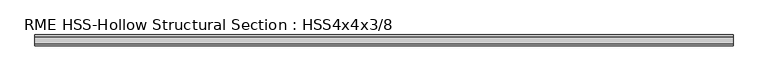
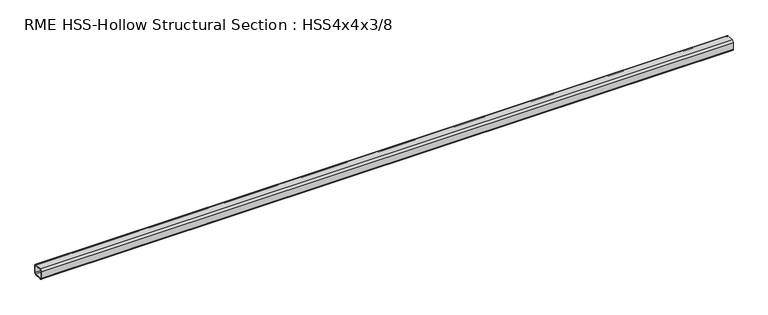
"""IFC4 building model written with IfcOpenShell, lengths in millimetres: member geometry, RME HSS-Hollow Structural Section : HSS4x4x3/8."""

from ifc_helpers import new_model, si_unit, point, frame, frame_2d, origin, place, context, project, spatial, polyline, circle_curve, trimmed, segment, composite_curve, outline, extrude, source, transform, mapped, element, save


def rme_hss_hollow_structural_section_hss4x4x3_8_4a4d7d68(model_context):
    return source(origin(), model_context, "Body", "SweptSolid", [
        extrude(outline(composite_curve([segment(polyline([(50.8, 33.0708), (50.8, -33.0708)]), True, "CONTINUOUS"), segment(trimmed(circle_curve(frame_2d((33.0708, -33.0708)), 17.7292), [point((50.8, -33.0708))], [point((33.0708, -50.8))], False, "CARTESIAN"), True, "CONTINUOUS"), segment(polyline([(33.0708, -50.8), (-33.0708, -50.8)]), True, "CONTINUOUS"), segment(trimmed(circle_curve(frame_2d((-33.0708, -33.0708)), 17.7292), [point((-33.0708, -50.8))], [point((-50.8, -33.0708))], False, "CARTESIAN"), True, "CONTINUOUS"), segment(polyline([(-50.8, -33.0708), (-50.8, 33.0708)]), True, "CONTINUOUS"), segment(trimmed(circle_curve(frame_2d((-33.0708, 33.0708)), 17.7292), [point((-50.8, 33.0708))], [point((-33.0708, 50.8))], False, "CARTESIAN"), True, "CONTINUOUS"), segment(polyline([(-33.0708, 50.8), (33.0708, 50.8)]), True, "CONTINUOUS"), segment(trimmed(circle_curve(frame_2d((33.0708, 33.0708)), 17.7292), [point((33.0708, 50.8))], [point((50.8, 33.0708))], False, "CARTESIAN"), True, "CONTINUOUS")], self_intersect=False), holes=[composite_curve([segment(trimmed(circle_curve(frame_2d((-33.0708, 33.0708)), 8.8646), [point((-33.0708, 41.9354))], [point((-41.9354, 33.0708))], True, "CARTESIAN"), True, "CONTINUOUS"), segment(polyline([(-41.9354, 33.0708), (-41.9354, -33.0708)]), True, "CONTINUOUS"), segment(trimmed(circle_curve(frame_2d((-33.0708, -33.0708)), 8.8646), [point((-41.9354, -33.0708))], [point((-33.0708, -41.9354))], True, "CARTESIAN"), True, "CONTINUOUS"), segment(polyline([(-33.0708, -41.9354), (33.0708, -41.9354)]), True, "CONTINUOUS"), segment(trimmed(circle_curve(frame_2d((33.0708, -33.0708)), 8.8646), [point((33.0708, -41.9354))], [point((41.9354, -33.0708))], True, "CARTESIAN"), True, "CONTINUOUS"), segment(polyline([(41.9354, -33.0708), (41.9354, 33.0708)]), True, "CONTINUOUS"), segment(trimmed(circle_curve(frame_2d((33.0708, 33.0708)), 8.8646), [point((41.9354, 33.0708))], [point((33.0708, 41.9354))], True, "CARTESIAN"), True, "CONTINUOUS"), segment(polyline([(33.0708, 41.9354), (-33.0708, 41.9354)]), True, "CONTINUOUS")], self_intersect=False)]), frame((-3369.3012077, 0.0, 0.0), z_axis=(1.0, 0.0, 0.0), x_axis=(0.0, 1.0, 0.0)), (0.0, 0.0, 1.0), 6538.9976176),
    ])


if __name__ == "__main__":
    model = new_model("IFC4")
    model_context = context("Model", 3, world=origin())
    ifc_project = project(units=[si_unit("LENGTHUNIT", "METRE", prefix="MILLI")], contexts=[model_context])
    site = spatial("IfcSite", under=ifc_project)
    building = spatial("IfcBuilding", under=site)
    placement = place(None, origin())
    rme_hss_hollow_structural_section_hss4x4x3_8_shape = rme_hss_hollow_structural_section_hss4x4x3_8_4a4d7d68(model_context)
    element("IfcMember", 1, ObjectType="RME HSS-Hollow Structural Section : HSS4x4x3/8", at=placement, inside=building, context=model_context, shape_type="MappedRepresentation", body=[
        mapped(rme_hss_hollow_structural_section_hss4x4x3_8_shape, transform((0.0, 0.0, 0.0), x_axis=(1.0, 0.0, 0.0), y_axis=(0.0, 1.0, 0.0), z_axis=(0.0, 0.0, 1.0))),
    ])
    save(model, "model.ifc")

# Revit data of these elements
# Type "RME HSS-Hollow Structural Section : HSS4x4x3/8"
#   Nominal Size = "HSS6x4"
#   Assembly Code = "B10"
#   Shape = "Square"
#   W = 17.2
#   Start Extension Calculation [instance default] = 10' - 0"
#   Start Extension [instance default] = -0' - 0 1/2"
#   End Extension Calculation [instance default] = 10' - 0"
#   End Extension [instance default] = -0' - 0 1/2"
#   Ht = 0' - 4"
#   Length [instance default] = 5' - 0"
#   b = 0' - 4"
#   kr = 0' - 0.698"
#   t = 0' - 0.349"
#   A = 0.0331944 SF
#   Structural Material [instance default] = Metal - Steel - ASTM A500 - Grade B - Rectangular and Square
# Element 1 (IfcMember, "RME HSS-Hollow Structural Section : HSS4x4x3/8")
#   Length = 23' - 10.37043"
#   Structural Material = Metal - Steel - ASTM A992
#   Materials on its faces: "Metal - Steel - ASTM A992"
# Materials
#   "Metal - Steel - ASTM A500 - Grade B - Rectangular and Square": class "Metal", colour RGB 255 128 0, transparency 0
#   "Metal - Steel - ASTM A992": class "Metal", colour RGB 255 128 0, transparency 0
